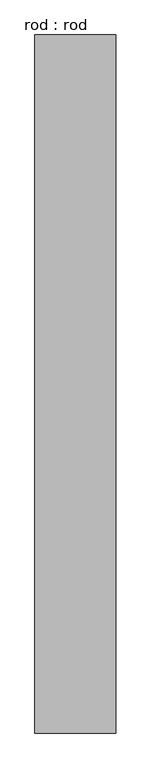
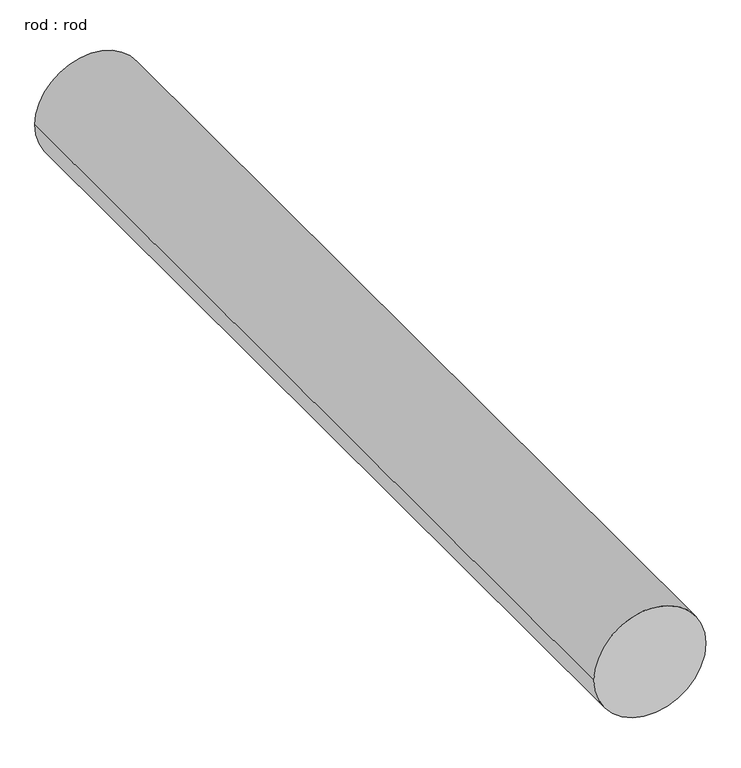
"""IFC4 building model written with IfcOpenShell, lengths in millimetres: proxy geometry, rod : rod."""

from ifc_helpers import new_model, si_unit, point, frame, frame_2d, origin, place, context, project, spatial, circle_curve, trimmed, segment, composite_curve, outline, extrude, source, transform, mapped, element, save


def rod_rod_c511721d(model_context):
    return source(origin(), model_context, "Body", "SweptSolid", [
        extrude(outline(composite_curve([segment(trimmed(circle_curve(frame_2d((0.0108462, 0.0)), 200.0), [point((0.0108462, 200.0))], [point((0.0108462, -200.0))], False, "CARTESIAN"), True, "CONTINUOUS"), segment(trimmed(circle_curve(frame_2d((0.0108462, 0.0)), 200.0), [point((0.0108462, -200.0))], [point((0.0108462, 200.0))], False, "CARTESIAN"), True, "CONTINUOUS")], self_intersect=False)), frame((0.0, 2362.3714725, 0.0), z_axis=(0.0, 1.0, 0.0), x_axis=(0.0, 0.0, 1.0)), (0.0, 0.0, 1.0), 3460.7142857),
    ])


if __name__ == "__main__":
    model = new_model("IFC4")
    model_context = context("Model", 3, world=origin())
    ifc_project = project(units=[si_unit("LENGTHUNIT", "METRE", prefix="MILLI")], contexts=[model_context])
    site = spatial("IfcSite", under=ifc_project)
    building = spatial("IfcBuilding", under=site)
    placement = place(None, origin())
    rod_rod_shape = rod_rod_c511721d(model_context)
    element("IfcBuildingElementProxy", 1, Name="rod : rod", ObjectType="rod : rod", at=placement, inside=building, context=model_context, shape_type="MappedRepresentation", body=[
        mapped(rod_rod_shape, transform((0.0, 0.0, 0.0), x_axis=(1.0, 0.0, 0.0), y_axis=(0.0, 1.0, 0.0), z_axis=(0.0, 0.0, 1.0))),
    ])
    save(model, "model.ifc")

# Revit data of these elements
# Type "rod : rod"
#   Default Elevation = 0
